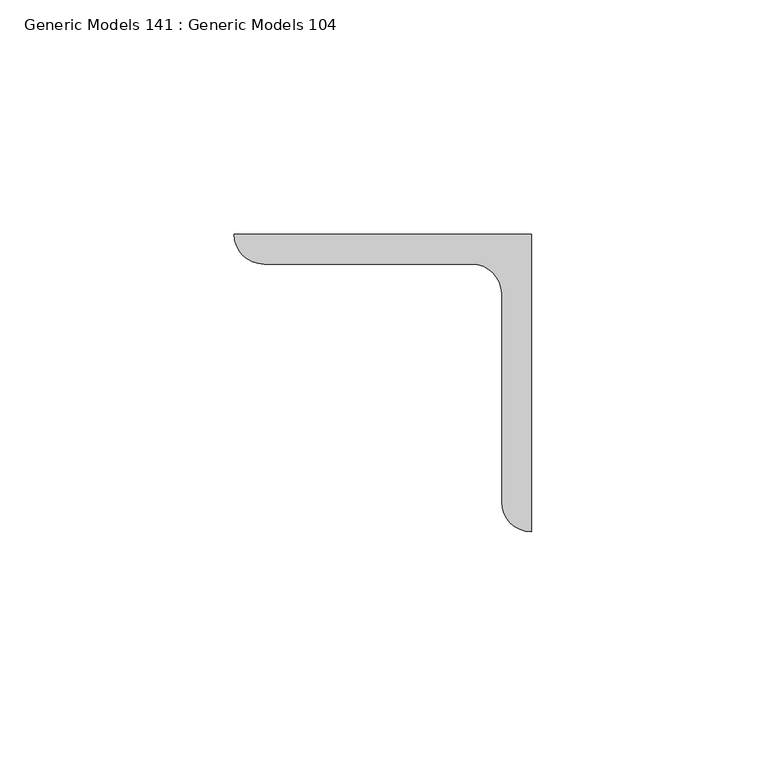
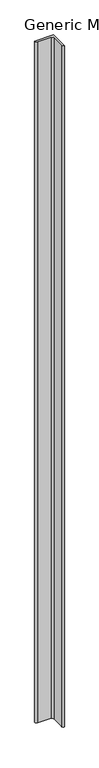
"""IFC4 building model written with IfcOpenShell, lengths in millimetres: proxy geometry, Generic Models 141 : Generic Models 104."""

from ifc_helpers import new_model, si_unit, point, frame, frame_2d, origin, place, context, project, spatial, polyline, circle_curve, trimmed, segment, composite_curve, outline, extrude, source, transform, mapped, element, save


def generic_models_141_generic_models_104_68167a8a(model_context):
    return source(origin(), model_context, "Body", "SweptSolid", [
        extrude(outline(composite_curve([segment(polyline([(32326.8940778, 41071.1196612), (32326.8940778, 41007.6196612)]), True, "CONTINUOUS"), segment(trimmed(circle_curve(frame_2d((32326.8940778, 41013.9696612)), 6.35), [point((32326.8940778, 41007.6196612))], [point((32320.5440778, 41013.9696612))], False, "CARTESIAN"), True, "CONTINUOUS"), segment(polyline([(32320.5440778, 41013.9696612), (32320.5440778, 41058.4196612)]), True, "CONTINUOUS"), segment(trimmed(circle_curve(frame_2d((32314.1940778, 41058.4196612)), 6.35), [point((32320.5440778, 41058.4196612))], [point((32314.1940778, 41064.7696612))], True, "CARTESIAN"), True, "CONTINUOUS"), segment(polyline([(32314.1940778, 41064.7696612), (32269.7440778, 41064.7696612)]), True, "CONTINUOUS"), segment(trimmed(circle_curve(frame_2d((32269.7440778, 41071.1196612)), 6.35), [point((32269.7440778, 41064.7696612))], [point((32263.3940778, 41071.1196612))], False, "CARTESIAN"), True, "CONTINUOUS"), segment(polyline([(32263.3940778, 41071.1196612), (32326.8940778, 41071.1196612)]), True, "CONTINUOUS")], self_intersect=False)), frame((0.0, 0.0, 266407.9), z_axis=(0.0, 0.0, 1.0), x_axis=(1.0, 0.0, 0.0)), (0.0, 0.0, 1.0), 2432.1044757),
    ])


if __name__ == "__main__":
    model = new_model("IFC4")
    model_context = context("Model", 3, world=origin())
    ifc_project = project(units=[si_unit("LENGTHUNIT", "METRE", prefix="MILLI")], contexts=[model_context])
    site = spatial("IfcSite", under=ifc_project)
    building = spatial("IfcBuilding", under=site)
    placement = place(None, origin())
    generic_models_141_generic_models_104_shape = generic_models_141_generic_models_104_68167a8a(model_context)
    element("IfcBuildingElementProxy", 1, Name="Generic Models 141 : Generic Models 104", ObjectType="Generic Models 141 : Generic Models 104", at=placement, inside=building, context=model_context, shape_type="MappedRepresentation", body=[
        mapped(generic_models_141_generic_models_104_shape, transform((0.0, 0.0, 0.0), x_axis=(1.0, 0.0, 0.0), y_axis=(0.0, 1.0, 0.0), z_axis=(0.0, 0.0, 1.0))),
    ])
    save(model, "model.ifc")

# Revit data of these elements
# Element 1 (IfcBuildingElementProxy, "Generic Models 141 : Generic Models 104")
#   Materials on its faces: "(2) BACK/BACK GALVANIZED ANGLES (2) L2 1/2 X 2 1/2 X 1/4\")"
# Materials
#   "(2) BACK/BACK GALVANIZED ANGLES (2) L2 1/2 X 2 1/2 X 1/4\")": class "Unassigned", colour RGB 211 211 211, transparency 0, Cost = 0
